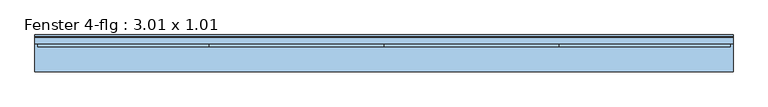
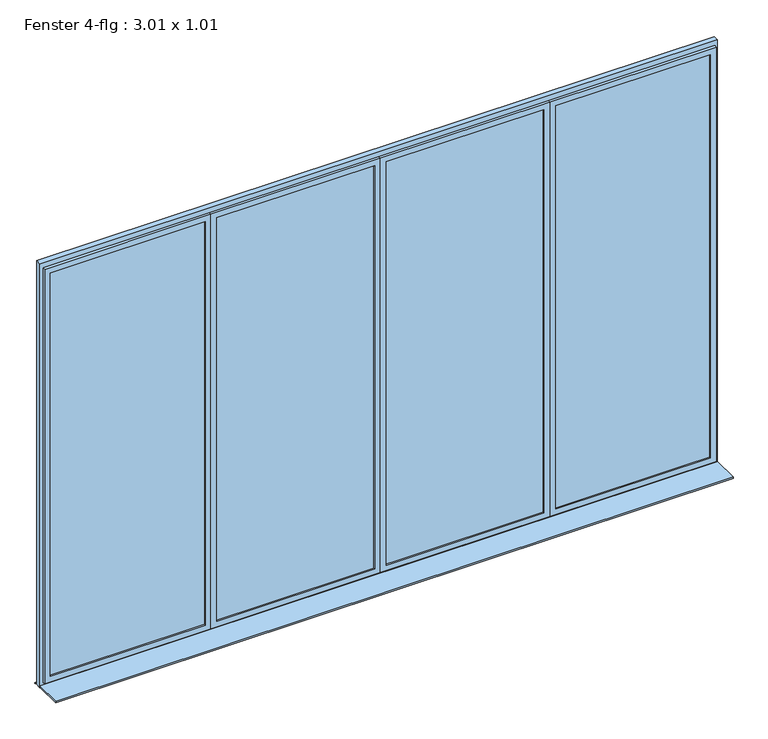
"""IFC4 building model written with IfcOpenShell, lengths in millimetres: window geometry, Fenster 4-flg : 3.01 x 1.01."""

from ifc_helpers import new_model, si_unit, frame, origin, place, context, project, spatial, polyline, outline, extrude, faceted_brep, source, transform, mapped, element, save


def fenster_4_flg_3_01_x_1_01_20ed2dc3(model_context):
    return source(origin(), model_context, "Body", "SolidModel", [
        extrude(outline(polyline([(4150.75, 155.0), (4150.75, 95.0), (4090.75, 95.0), (4090.75, 155.0), (4150.75, 155.0)])), frame((0.0, 0.0, 1080.0), z_axis=(0.0, 0.0, 1.0), x_axis=(1.0, 0.0, 0.0)), (0.0, 0.0, 1.0), 4470.0),
        extrude(outline(polyline([(2400.5, 155.0), (2400.5, 95.0), (2340.5, 95.0), (2340.5, 155.0), (2400.5, 155.0)])), frame((0.0, 0.0, 1080.0), z_axis=(0.0, 0.0, 1.0), x_axis=(1.0, 0.0, 0.0)), (0.0, 0.0, 1.0), 4470.0),
        extrude(outline(polyline([(650.25, 155.0), (650.25, 95.0), (590.25, 95.0), (590.25, 155.0), (650.25, 155.0)])), frame((0.0, 0.0, 1080.0), z_axis=(0.0, 0.0, 1.0), x_axis=(1.0, 0.0, 0.0)), (0.0, 0.0, 1.0), 4470.0),
        extrude(outline(polyline([(5630.0, 5871.0), (5630.0, -1130.0), (1000.0, -1130.0), (1000.0, 5871.0), (5630.0, 5871.0)]), holes=[polyline([(5550.0, 5811.0), (1080.0, 5811.0), (1080.0, -1070.0), (5550.0, -1070.0), (5550.0, 5811.0)])]), frame((0.0, 95.0, 0.0), z_axis=(0.0, 1.0, 0.0), x_axis=(0.0, 0.0, 1.0)), (0.0, 0.0, 1.0), 60.0),
        faceted_brep([(4120.75, 95.0, 5580.0), (4120.75, 65.0, 5580.0), (4120.75, 65.0, 1050.0), (4120.75, 95.0, 1050.0), (2370.5, 65.0, 5580.0), (2370.5, 65.0, 1050.0), (4060.75, 65.0, 1110.0), (2430.5, 65.0, 1110.0), (2430.5, 65.0, 5520.0), (4060.75, 65.0, 5520.0), (2370.5, 95.0, 1050.0), (2370.5, 95.0, 5580.0), (4090.75, 95.0, 5550.0), (2400.5, 95.0, 5550.0), (2400.5, 95.0, 1080.0), (4090.75, 95.0, 1080.0), (4090.75, 125.0, 5550.0), (4090.75, 125.0, 1080.0), (2400.5, 125.0, 1080.0), (2400.5, 125.0, 5550.0), (4060.75, 125.0, 5520.0), (2430.5, 125.0, 5520.0), (2430.5, 125.0, 1110.0), (4060.75, 125.0, 1110.0)], [[[0, 1, 2, 3]], [[1, 4, 5, 2], [6, 7, 8, 9]], [[3, 2, 5, 10]], [[3, 10, 11, 0], [12, 13, 14, 15]], [[16, 12, 15, 17]], [[17, 15, 14, 18]], [[17, 18, 19, 16], [20, 21, 22, 23]], [[9, 20, 23, 6]], [[6, 23, 22, 7]], [[10, 5, 4, 11]], [[18, 14, 13, 19]], [[7, 22, 21, 8]], [[11, 4, 1, 0]], [[19, 13, 12, 16]], [[8, 21, 20, 9]]]),
        faceted_brep([(2370.5, 95.0, 5580.0), (2370.5, 65.0, 5580.0), (2370.5, 65.0, 1050.0), (2370.5, 95.0, 1050.0), (620.25, 65.0, 5580.0), (620.25, 65.0, 1050.0), (2310.5, 65.0, 1110.0), (680.25, 65.0, 1110.0), (680.25, 65.0, 5520.0), (2310.5, 65.0, 5520.0), (620.25, 95.0, 1050.0), (620.25, 95.0, 5580.0), (2340.5, 95.0, 5550.0), (650.25, 95.0, 5550.0), (650.25, 95.0, 1080.0), (2340.5, 95.0, 1080.0), (2340.5, 125.0, 5550.0), (2340.5, 125.0, 1080.0), (650.25, 125.0, 1080.0), (650.25, 125.0, 5550.0), (2310.5, 125.0, 5520.0), (680.25, 125.0, 5520.0), (680.25, 125.0, 1110.0), (2310.5, 125.0, 1110.0)], [[[0, 1, 2, 3]], [[1, 4, 5, 2], [6, 7, 8, 9]], [[3, 2, 5, 10]], [[3, 10, 11, 0], [12, 13, 14, 15]], [[16, 12, 15, 17]], [[17, 15, 14, 18]], [[17, 18, 19, 16], [20, 21, 22, 23]], [[9, 20, 23, 6]], [[6, 23, 22, 7]], [[10, 5, 4, 11]], [[18, 14, 13, 19]], [[7, 22, 21, 8]], [[11, 4, 1, 0]], [[19, 13, 12, 16]], [[8, 21, 20, 9]]]),
        faceted_brep([(620.25, 95.0, 5580.0), (620.25, 65.0, 5580.0), (620.25, 65.0, 1050.0), (620.25, 95.0, 1050.0), (-1100.0, 65.0, 5580.0), (-1100.0, 65.0, 1050.0), (560.25, 65.0, 1110.0), (-1040.0, 65.0, 1110.0), (-1040.0, 65.0, 5520.0), (560.25, 65.0, 5520.0), (-1100.0, 95.0, 1050.0), (-1100.0, 95.0, 5580.0), (590.25, 95.0, 5550.0), (-1070.0, 95.0, 5550.0), (-1070.0, 95.0, 1080.0), (590.25, 95.0, 1080.0), (590.25, 125.0, 5550.0), (590.25, 125.0, 1080.0), (-1070.0, 125.0, 1080.0), (-1070.0, 125.0, 5550.0), (560.25, 125.0, 5520.0), (-1040.0, 125.0, 5520.0), (-1040.0, 125.0, 1110.0), (560.25, 125.0, 1110.0)], [[[0, 1, 2, 3]], [[1, 4, 5, 2], [6, 7, 8, 9]], [[3, 2, 5, 10]], [[3, 10, 11, 0], [12, 13, 14, 15]], [[16, 12, 15, 17]], [[17, 15, 14, 18]], [[17, 18, 19, 16], [20, 21, 22, 23]], [[9, 20, 23, 6]], [[6, 23, 22, 7]], [[10, 5, 4, 11]], [[18, 14, 13, 19]], [[7, 22, 21, 8]], [[11, 4, 1, 0]], [[19, 13, 12, 16]], [[8, 21, 20, 9]]]),
        faceted_brep([(5841.0, 95.0, 5580.0), (5841.0, 65.0, 5580.0), (5841.0, 65.0, 1050.0), (5841.0, 95.0, 1050.0), (4120.75, 65.0, 5580.0), (4120.75, 65.0, 1050.0), (5781.0, 65.0, 1110.0), (4180.75, 65.0, 1110.0), (4180.75, 65.0, 5520.0), (5781.0, 65.0, 5520.0), (4120.75, 95.0, 1050.0), (4120.75, 95.0, 5580.0), (5811.0, 95.0, 5550.0), (4150.75, 95.0, 5550.0), (4150.75, 95.0, 1080.0), (5811.0, 95.0, 1080.0), (5811.0, 125.0, 5550.0), (5811.0, 125.0, 1080.0), (4150.75, 125.0, 1080.0), (4150.75, 125.0, 5550.0), (5781.0, 125.0, 5520.0), (4180.75, 125.0, 5520.0), (4180.75, 125.0, 1110.0), (5781.0, 125.0, 1110.0)], [[[0, 1, 2, 3]], [[1, 4, 5, 2], [6, 7, 8, 9]], [[3, 2, 5, 10]], [[3, 10, 11, 0], [12, 13, 14, 15]], [[16, 12, 15, 17]], [[17, 15, 14, 18]], [[17, 18, 19, 16], [20, 21, 22, 23]], [[9, 20, 23, 6]], [[6, 23, 22, 7]], [[10, 5, 4, 11]], [[18, 14, 13, 19]], [[7, 22, 21, 8]], [[11, 4, 1, 0]], [[19, 13, 12, 16]], [[8, 21, 20, 9]]]),
        extrude(outline(polyline([(165.0221543, 1020.0), (185.0, 1000.0), (185.0, 990.0), (183.0, 990.0), (183.0, 998.3604634), (164.8240723, 1018.0), (155.0, 1018.0), (155.0, 1020.0), (165.0221543, 1020.0)])), frame((-1130.0, 0.0, 0.0), z_axis=(1.0, 0.0, 0.0), x_axis=(0.0, 1.0, 0.0)), (0.0, 0.0, 1.0), 7001.0),
        extrude(outline(polyline([(-1130.0, -185.0), (-1130.0, 95.0), (5871.0, 95.0), (5871.0, -185.0), (-1130.0, -185.0)])), frame((0.0, 0.0, 1005.0), z_axis=(0.0, 0.0, 1.0), x_axis=(1.0, 0.0, 0.0)), (0.0, 0.0, 1.0), 15.0),
        extrude(outline(polyline([(560.25, 80.0), (-1040.0, 80.0), (-1040.0, 110.0), (560.25, 110.0), (560.25, 80.0)])), frame((0.0, 0.0, 1110.0), z_axis=(0.0, 0.0, 1.0), x_axis=(1.0, 0.0, 0.0)), (0.0, 0.0, 1.0), 4410.0),
        extrude(outline(polyline([(2310.5, 80.0), (680.25, 80.0), (680.25, 110.0), (2310.5, 110.0), (2310.5, 80.0)])), frame((0.0, 0.0, 1110.0), z_axis=(0.0, 0.0, 1.0), x_axis=(1.0, 0.0, 0.0)), (0.0, 0.0, 1.0), 4410.0),
        extrude(outline(polyline([(4060.75, 80.0), (2430.5, 80.0), (2430.5, 110.0), (4060.75, 110.0), (4060.75, 80.0)])), frame((0.0, 0.0, 1110.0), z_axis=(0.0, 0.0, 1.0), x_axis=(1.0, 0.0, 0.0)), (0.0, 0.0, 1.0), 4410.0),
        extrude(outline(polyline([(5781.0, 80.0), (4180.75, 80.0), (4180.75, 110.0), (5781.0, 110.0), (5781.0, 80.0)])), frame((0.0, 0.0, 1110.0), z_axis=(0.0, 0.0, 1.0), x_axis=(1.0, 0.0, 0.0)), (0.0, 0.0, 1.0), 4410.0),
    ])


if __name__ == "__main__":
    model = new_model("IFC4")
    model_context = context("Model", 3, world=origin())
    ifc_project = project(units=[si_unit("LENGTHUNIT", "METRE", prefix="MILLI")], contexts=[model_context])
    site = spatial("IfcSite", under=ifc_project)
    building = spatial("IfcBuilding", under=site)
    placement = place(None, origin())
    fenster_4_flg_3_01_x_1_01_shape = fenster_4_flg_3_01_x_1_01_20ed2dc3(model_context)
    element("IfcWindow", 1, ObjectType="Fenster 4-flg : 3.01 x 1.01", at=placement, inside=building, context=model_context, shape_type="MappedRepresentation", body=[
        mapped(fenster_4_flg_3_01_x_1_01_shape, transform((0.0, 0.0, 0.0), x_axis=(1.0, 0.0, 0.0), y_axis=(0.0, 1.0, 0.0), z_axis=(0.0, 0.0, 1.0))),
    ])
    save(model, "model.ifc")

# Revit data of these elements
# Type "Fenster 4-flg : 3.01 x 1.01"
#   Type Mark = "51"
#   Operation = "UserDefined"
#   Keynote = "16.05.01"
#   Visual Light Transmittance = 0.9
#   Solar Heat Gain Coefficient = 0.78
#   Rough Height = 4.630 m
#   Rough Width = 7.001 m
#   Heat Transfer Coefficient (U) = 3.6886 W/(m²·K)
#   Rahmentiefe = 0.060 m
#   Breite unterer Rahmen = 0.080 m
#   Breite oberer  Rahmen = 0.080 m
#   Rahmenbreite = 0.060 m
#   Height = 4.630 m
#   Tiefe Flügel = 0.060 m
#   Flügelbreite = 0.060 m
#   Einbautiefe (von außen) [instance default] = 0.080 m
#   Width = 7.001 m
#   Bild = Metall - Aluminium
#   Glas = Fenster - Glas
#   Fensterflügel = Metall - Aluminium
#   Innere Fensterbank = Metall - Aluminium
#   Äußere Fensterbank = Metall - Aluminium
#   Construction Type Id = ""
#   Wall Closure = (empty or 0)
#   Analytic Construction = (empty or 0)
# Element 1 (IfcWindow, "Fenster 4-flg : 3.01 x 1.01")
#   Einbautiefe (von außen) = 0.000 m
#   Materials on its faces: "Metall - Aluminium", "Fenster - Glas"
# Materials
#   "Metall - Aluminium": class "Metall", colour RGB 247 247 247, transparency 0, Description = "Aluminium 6061", Cost = 0
#   "Fenster - Glas": class "Glas", colour RGB 128 128 255, transparency 0.75, Cost = 0
